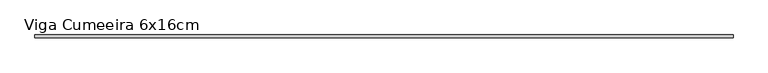
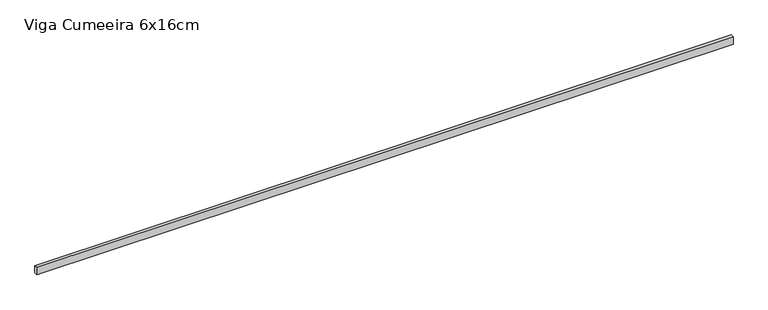
"""IFC4 building model written with IfcOpenShell, lengths in millimetres: beam geometry, Madeira de lei : Viga Cumeeira 6x16cm."""

from ifc_helpers import new_model, si_unit, frame, origin, place, context, project, spatial, polyline, outline, extrude, source, transform, mapped, element, save


def viga_cumeeira_6x16cm_bb341ce4(model_context):
    return source(origin(), model_context, "Body", "SweptSolid", [
        extrude(outline(polyline([(7083.3, 30.0), (7083.3, -30.0), (-7082.5, -30.0), (-7082.5, 30.0), (7083.3, 30.0)])), frame((0.0, 0.0, -80.0), z_axis=(0.0, 0.0, 1.0), x_axis=(1.0, 0.0, 0.0)), (0.0, 0.0, 1.0), 160.0),
    ])


if __name__ == "__main__":
    model = new_model("IFC4")
    model_context = context("Model", 3, world=origin())
    ifc_project = project(units=[si_unit("LENGTHUNIT", "METRE", prefix="MILLI")], contexts=[model_context])
    site = spatial("IfcSite", under=ifc_project)
    building = spatial("IfcBuilding", under=site)
    placement = place(None, origin())
    viga_cumeeira_6x16cm_shape = viga_cumeeira_6x16cm_bb341ce4(model_context)
    element("IfcBeam", 1, ObjectType="Madeira de lei : Viga Cumeeira 6x16cm", at=placement, inside=building, context=model_context, shape_type="MappedRepresentation", body=[
        mapped(viga_cumeeira_6x16cm_shape, transform((0.0, 0.0, 0.0), x_axis=(1.0, 0.0, 0.0), y_axis=(0.0, 1.0, 0.0), z_axis=(0.0, 0.0, 1.0))),
    ])
    save(model, "model.ifc")

# Revit data of these elements
# Type "Madeira de lei : Viga Cumeeira 6x16cm"
#   A = 0.02 m²
#   Length [instance default] = 1.524 m
#   b = 0.06 m
#   d = 0.16 m
#   Structural Material [instance default] = none
#   Assembly Code = ""
# Element 1 (IfcBeam, "Madeira de lei : Viga Cumeeira 6x16cm")
#   Structural Material = .MADEIRAMENTO
#   Materials on its faces: ".MADEIRAMENTO"
# Materials
#   ".MADEIRAMENTO": class ".CC_MADEIRAS", colour RGB 212 179 113, transparency 0, Cost = 0
